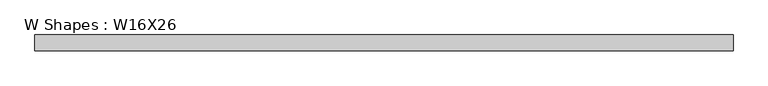
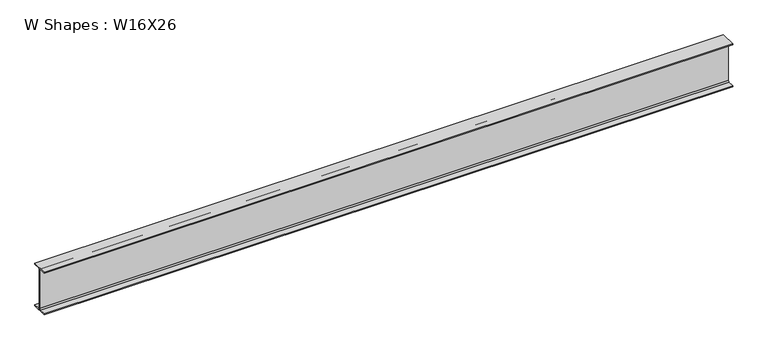
"""IFC4 building model written with IfcOpenShell, lengths in millimetres: beam geometry, W Shapes : W16X26."""

from ifc_helpers import new_model, si_unit, point, frame, frame_2d, origin, place, context, project, spatial, polyline, circle_curve, trimmed, segment, composite_curve, outline, extrude, source, transform, mapped, element, save


def w_shapes_w16x26_047c9101(model_context):
    return source(origin(), model_context, "Body", "SweptSolid", [
        extrude(outline(composite_curve([segment(polyline([(69.85, -190.627), (69.85, -199.39), (-69.85, -199.39), (-69.85, -190.627), (-13.3858, -190.627)]), True, "CONTINUOUS"), segment(trimmed(circle_curve(frame_2d((-13.3858, -180.4162)), 10.2108), [point((-13.3858, -190.627))], [point((-3.175, -180.4162))], True, "CARTESIAN"), True, "CONTINUOUS"), segment(polyline([(-3.175, -180.4162), (-3.175, 180.4162)]), True, "CONTINUOUS"), segment(trimmed(circle_curve(frame_2d((-13.3858, 180.4162)), 10.2108), [point((-3.175, 180.4162))], [point((-13.3858, 190.627))], True, "CARTESIAN"), True, "CONTINUOUS"), segment(polyline([(-13.3858, 190.627), (-69.85, 190.627), (-69.85, 199.39), (69.85, 199.39), (69.85, 190.627), (13.3858, 190.627)]), True, "CONTINUOUS"), segment(trimmed(circle_curve(frame_2d((13.3858, 180.4162)), 10.2108), [point((13.3858, 190.627))], [point((3.175, 180.4162))], True, "CARTESIAN"), True, "CONTINUOUS"), segment(polyline([(3.175, 180.4162), (3.175, -180.4162)]), True, "CONTINUOUS"), segment(trimmed(circle_curve(frame_2d((13.3858, -180.4162)), 10.2108), [point((3.175, -180.4162))], [point((13.3858, -190.627))], True, "CARTESIAN"), True, "CONTINUOUS"), segment(polyline([(13.3858, -190.627), (69.85, -190.627)]), True, "CONTINUOUS")], self_intersect=False)), frame((-3048.0, 0.0, 0.0), z_axis=(1.0, 0.0, 0.0), x_axis=(0.0, 1.0, 0.0)), (0.0, 0.0, 1.0), 6096.0),
    ])


if __name__ == "__main__":
    model = new_model("IFC4")
    model_context = context("Model", 3, world=origin())
    ifc_project = project(units=[si_unit("LENGTHUNIT", "METRE", prefix="MILLI")], contexts=[model_context])
    site = spatial("IfcSite", under=ifc_project)
    building = spatial("IfcBuilding", under=site)
    placement = place(None, origin())
    w_shapes_w16x26_shape = w_shapes_w16x26_047c9101(model_context)
    element("IfcBeam", 1, ObjectType="W Shapes : W16X26", at=placement, inside=building, context=model_context, shape_type="MappedRepresentation", body=[
        mapped(w_shapes_w16x26_shape, transform((0.0, 0.0, 0.0), x_axis=(1.0, 0.0, 0.0), y_axis=(0.0, 1.0, 0.0), z_axis=(0.0, 0.0, 1.0))),
    ])
    save(model, "model.ifc")

# Revit data of these elements
# Type "W Shapes : W16X26"
#   Section Name Key = "W16x26"
#   Assembly Code = "B10"
#   Width = 5.500"
#   Web Thickness = 0.250"
#   Web Fillet = 0.402"
#   Warping Constant = 565.00 in⁶
#   Torsional Moment of Inertia = 0.262 in⁴
#   Section Area = 7.68 in²
#   Plastic Modulus weak axis = 5.48 in³
#   Plastic Modulus strong axis = 44.20 in³
#   Perimeter = 4.35 ft²/ft
#   Nominal Weight = 26.00 lbf/ft
#   Moment of Inertia weak axis = 9.59 in⁴
#   Moment of Inertia strong axis = 301.00 in⁴
#   Height = 15.700"
#   Flange Thickness = 0.345"
#   Elastic Modulus weak axis = 3.49 in³
#   Elastic Modulus strong axis = 38.40 in³
#   Centroid Vertical = 7.850"
#   Centroid Horizontal = 2.750"
#   Bolt Spacing = 0' - 3 1/2"
#   Length [instance default] = 5' - 0"
#   Structural Material [instance default] = Steel ASTM A992
#   Principal Axes Angle = 0
# Element 1 (IfcBeam, "W Shapes : W16X26")
#   Structural Material = Steel ASTM A36
#   Materials on its faces: "Steel ASTM A36"
# Materials
#   "Steel ASTM A992": class "Metal", colour RGB 199 199 199, transparency 0, Description = "Structural steel 50ksi", Cost = 0
#   "Steel ASTM A36": class "Metal", colour RGB 199 199 199, transparency 0, Description = "Structural steel, ASTM A36 Grade B, mill finish", Cost = 0
